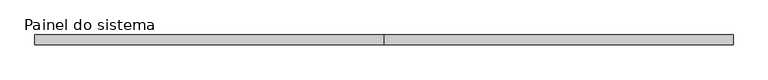
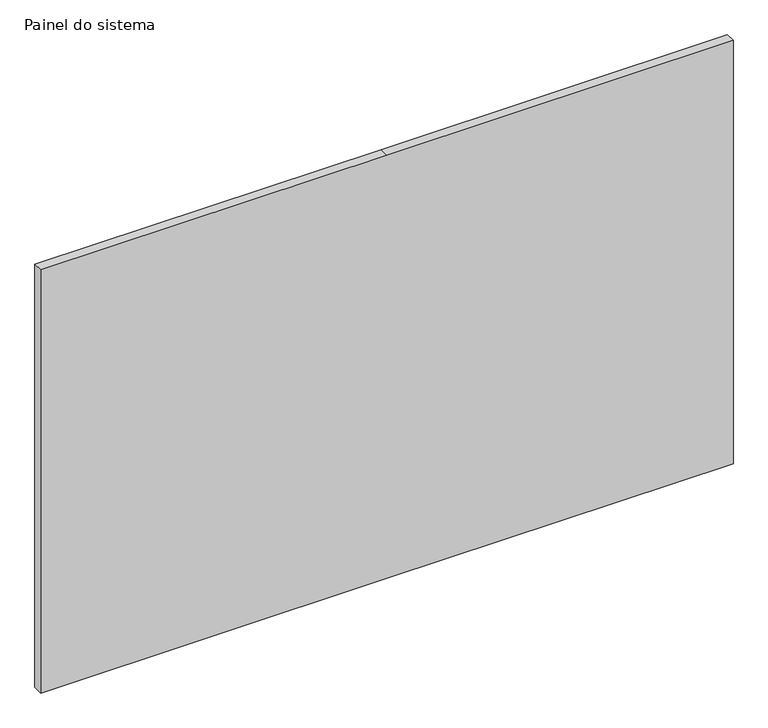
"""IFC4 building model written with IfcOpenShell, lengths in millimetres: plate geometry, Painel do sistema : Envidraçado."""

from ifc_helpers import new_model, si_unit, frame, origin, place, context, project, spatial, polyline, outline, extrude, source, transform, mapped, element, save


def painel_do_sistema_d3c51492(model_context):
    return source(origin(), model_context, "Body", "SweptSolid", [
        extrude(outline(polyline([(0.0, -890.0), (0.0, 0.0), (0.0, 890.0), (1150.0, 890.0), (1150.0, 0.0), (1150.0, -890.0), (0.0, -890.0)])), frame((0.0, 24.5, 0.0), z_axis=(0.0, 1.0, 0.0), x_axis=(0.0, 0.0, 1.0)), (0.0, 0.0, 1.0), 25.0),
    ])


if __name__ == "__main__":
    model = new_model("IFC4")
    model_context = context("Model", 3, world=origin())
    ifc_project = project(units=[si_unit("LENGTHUNIT", "METRE", prefix="MILLI")], contexts=[model_context])
    site = spatial("IfcSite", under=ifc_project)
    building = spatial("IfcBuilding", under=site)
    placement = place(None, origin())
    painel_do_sistema_shape = painel_do_sistema_d3c51492(model_context)
    element("IfcPlate", 1, ObjectType="Painel do sistema : Envidraçado", at=placement, inside=building, context=model_context, shape_type="MappedRepresentation", body=[
        mapped(painel_do_sistema_shape, transform((0.0, 0.0, 0.0), x_axis=(1.0, 0.0, 0.0), y_axis=(0.0, 1.0, 0.0), z_axis=(0.0, 0.0, 1.0))),
    ])
    save(model, "model.ifc")

# Revit data of these elements
# Type "Painel do sistema : Envidraçado"
#   Construction Type Id = "GSP4R"
#   Analytic Construction = "Vidraça única Pilkington 1/8 pol"
#   Visual Light Transmittance = 0.9
#   Solar Heat Gain Coefficient = 0.86
#   Heat Transfer Coefficient (U) = 6.7069 W/(m²·K)
# Element 1 (IfcPlate, "Painel do sistema : Envidraçado")
#   Materials on its faces: "Vidro"
# Materials
#   "Vidro": class "Vidro", colour RGB 0 128 192, transparency 0.9, Description = "Vidro de sílica", Cost = 0
